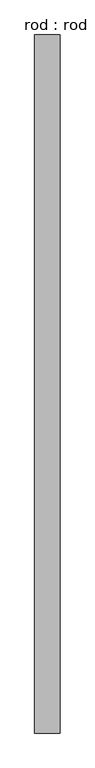
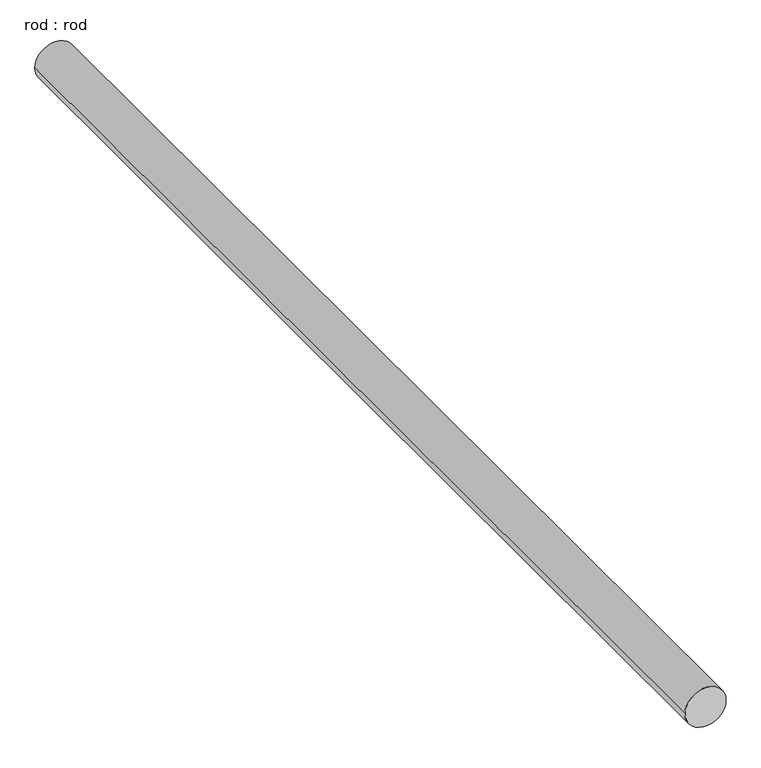
"""IFC4 building model written with IfcOpenShell, lengths in millimetres: proxy geometry, rod : rod."""

from ifc_helpers import new_model, si_unit, point, frame, frame_2d, origin, place, context, project, spatial, circle_curve, trimmed, segment, composite_curve, outline, extrude, source, transform, mapped, element, save


def rod_rod_a62a0fbd(model_context):
    return source(origin(), model_context, "Body", "SweptSolid", [
        extrude(outline(composite_curve([segment(trimmed(circle_curve(frame_2d((0.0108462, 0.0)), 200.0), [point((0.0108462, 200.0))], [point((0.0108462, -200.0))], False, "CARTESIAN"), True, "CONTINUOUS"), segment(trimmed(circle_curve(frame_2d((0.0108462, 0.0)), 200.0), [point((0.0108462, -200.0))], [point((0.0108462, 200.0))], False, "CARTESIAN"), True, "CONTINUOUS")], self_intersect=False)), frame((0.0, -1407.2713847, 0.0), z_axis=(0.0, 1.0, 0.0), x_axis=(0.0, 0.0, 1.0)), (0.0, 0.0, 1.0), 11000.0),
    ])


if __name__ == "__main__":
    model = new_model("IFC4")
    model_context = context("Model", 3, world=origin())
    ifc_project = project(units=[si_unit("LENGTHUNIT", "METRE", prefix="MILLI")], contexts=[model_context])
    site = spatial("IfcSite", under=ifc_project)
    building = spatial("IfcBuilding", under=site)
    placement = place(None, origin())
    rod_rod_shape = rod_rod_a62a0fbd(model_context)
    element("IfcBuildingElementProxy", 1, Name="rod : rod", ObjectType="rod : rod", at=placement, inside=building, context=model_context, shape_type="MappedRepresentation", body=[
        mapped(rod_rod_shape, transform((0.0, 0.0, 0.0), x_axis=(1.0, 0.0, 0.0), y_axis=(0.0, 1.0, 0.0), z_axis=(0.0, 0.0, 1.0))),
    ])
    save(model, "model.ifc")

# Revit data of these elements
# Type "rod : rod"
#   Default Elevation = 0
